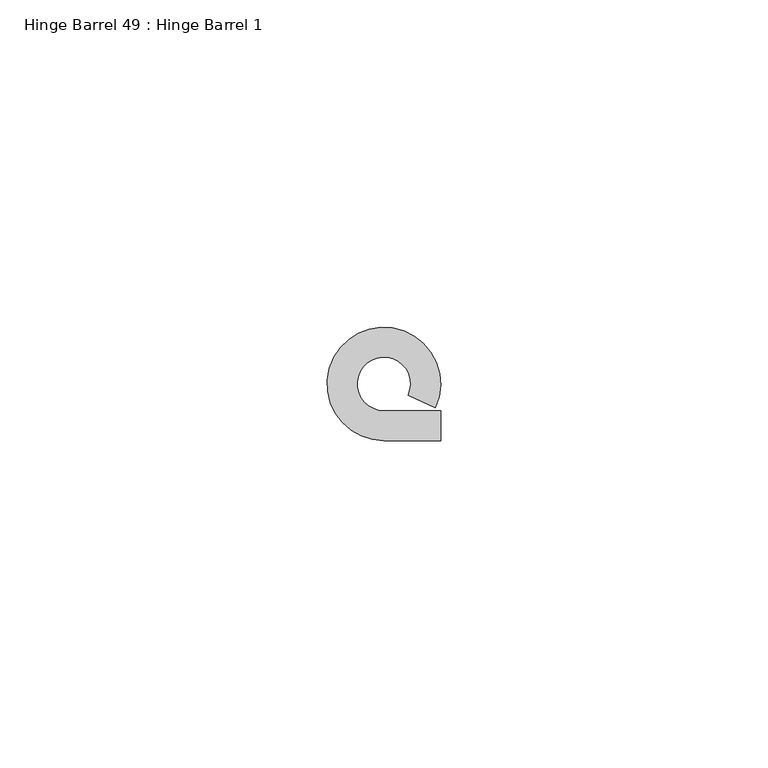
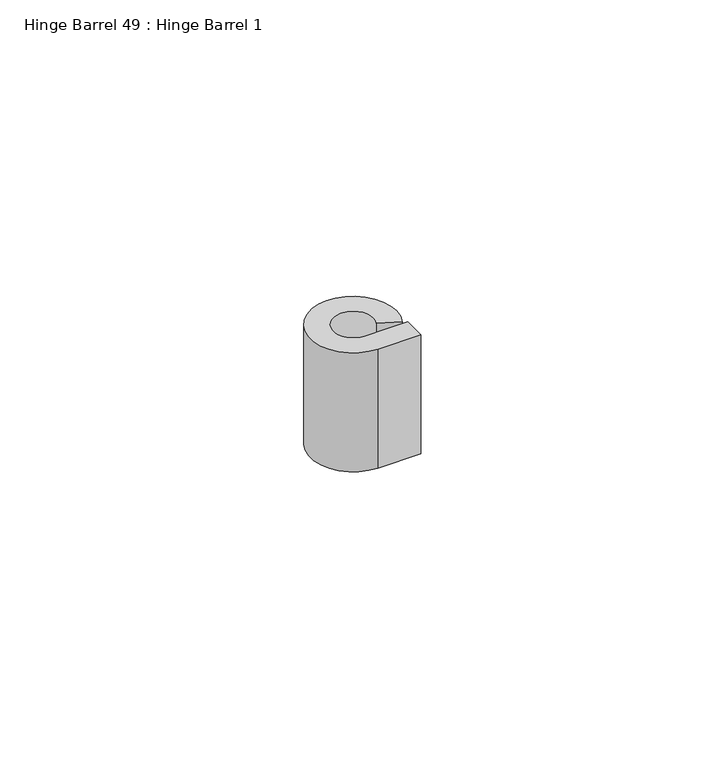
"""IFC4 building model written with IfcOpenShell, lengths in millimetres: proxy geometry, Hinge Barrel 49 : Hinge Barrel 1."""

import ifcopenshell
import ifcopenshell.guid

model = None  # the IFC model being written
_history = None  # IfcOwnerHistory: only IFC2X3 demands one
_inside = {}  # id of a spatial element -> (the spatial element, [elements in it])
_under = {}  # id of a project, library or spatial element -> (it, [spatial elements below it])
_declared = {}  # id of a project -> (the project, [libraries it declares])
_typed = {}  # id of a type object -> (the type object, [elements of that type])
_made_of = {}  # id of a material, layer set ... -> (it, [elements and type objects made of it])


def new_model(schema):
    """Start an empty IFC model of exactly this schema.

    Asked for "IFC4X3", IfcOpenShell would pick the latest addendum, in which some entities
    have other attributes; the version numbers below select the first issue.
    IFC2X3 requires an IfcOwnerHistory on every rooted entity: one is made here for all.
    """
    global model, _history
    if schema == "IFC4X3":
        model = ifcopenshell.file(schema_version=(4, 3, 0, 0))
    else:
        model = ifcopenshell.file(schema=schema)
    _inside.clear()
    _under.clear()
    _declared.clear()
    _typed.clear()
    _made_of.clear()
    _history = None
    if model.schema == "IFC2X3":
        org = make("IfcOrganization", Name="unknown")
        user = make(
            "IfcPersonAndOrganization",
            ThePerson=make("IfcPerson", FamilyName="unknown"),
            TheOrganization=org,
        )
        app = make(
            "IfcApplication",
            ApplicationDeveloper=org,
            Version="unknown",
            ApplicationFullName="unknown",
            ApplicationIdentifier="unknown",
        )
        _history = make(
            "IfcOwnerHistory",
            OwningUser=user,
            OwningApplication=app,
            ChangeAction="ADDED",
            CreationDate=0,
        )
    return model


def make(cls, **values):
    """One entity of the class cls with the attributes given. An attribute that is None is left unset."""
    return model.create_entity(
        cls, **{name: value for name, value in values.items() if value is not None}
    )


def rooted(cls, **values):
    """An entity with a GlobalId (a new one), such as an element, a storey or a relation."""
    return make(cls, GlobalId=ifcopenshell.guid.new(), OwnerHistory=_history, **values)


def si_unit(unit_type, name, prefix=None):
    """IfcSIUnit, for example si_unit("LENGTHUNIT", "METRE", prefix="MILLI")."""
    return make("IfcSIUnit", UnitType=unit_type, Prefix=prefix, Name=name)


def assignment(units):
    """IfcUnitAssignment: the units of a project."""
    return None if units is None else make("IfcUnitAssignment", Units=units)


def point(xyz):
    """IfcCartesianPoint."""
    return None if xyz is None else make("IfcCartesianPoint", Coordinates=xyz)


def direction(xyz):
    """IfcDirection."""
    return None if xyz is None else make("IfcDirection", DirectionRatios=xyz)


def frame(location, z_axis=None, x_axis=None):
    """IfcAxis2Placement3D, a coordinate frame: its origin and axes. An axis left out is left unset."""
    return make(
        "IfcAxis2Placement3D",
        Location=point(location),
        Axis=direction(z_axis),
        RefDirection=direction(x_axis),
    )


def frame_2d(location, x_axis=None):
    """IfcAxis2Placement2D, a coordinate frame in the plane: its origin and x axis."""
    return make(
        "IfcAxis2Placement2D", Location=point(location), RefDirection=direction(x_axis)
    )


def origin():
    """The frame at (0, 0, 0) with its axes left unset."""
    return frame((0.0, 0.0, 0.0))


def place(relative_to, where):
    """IfcLocalPlacement: puts the frame where relative to a parent placement (None: the world)."""
    return make(
        "IfcLocalPlacement", PlacementRelTo=relative_to, RelativePlacement=where
    )


def context(
    kind, dimensions, precision=None, world=None, true_north=None, identifier=None
):
    """IfcGeometricRepresentationContext, for example the 3D "Model" context."""
    return make(
        "IfcGeometricRepresentationContext",
        ContextIdentifier=identifier,
        ContextType=kind,
        CoordinateSpaceDimension=dimensions,
        Precision=precision,
        WorldCoordinateSystem=world,
        TrueNorth=true_north,
    )


def project(units=None, contexts=None):
    """IfcProject with its units and contexts."""
    return rooted(
        "IfcProject",
        Name="project",
        RepresentationContexts=contexts,
        UnitsInContext=assignment(units),
    )


def spatial(cls, under=None, at=None, **own):
    """A site, building, storey or space (cls), placed at a placement, below another one or the project."""
    s = rooted(cls, ObjectPlacement=at, **own)
    if under is not None:
        _under.setdefault(under.id(), (under, []))[1].append(s)
    return s


def polyline(points):
    """IfcPolyline through the points."""
    return make("IfcPolyline", Points=[point(p) for p in points])


def circle_curve(where, radius):
    """IfcCircle in the frame where."""
    return make("IfcCircle", Position=where, Radius=radius)


def trimmed(basis, trim1, trim2, sense, master):
    """IfcTrimmedCurve: the piece of a basis curve between two trims."""
    return make(
        "IfcTrimmedCurve",
        BasisCurve=basis,
        Trim1=trim1,
        Trim2=trim2,
        SenseAgreement=sense,
        MasterRepresentation=master,
    )


def segment(curve, same_sense, transition):
    """IfcCompositeCurveSegment."""
    return make(
        "IfcCompositeCurveSegment",
        Transition=transition,
        SameSense=same_sense,
        ParentCurve=curve,
    )


def composite_curve(segments, self_intersect=None):
    """IfcCompositeCurve: segments joined end to end."""
    return make("IfcCompositeCurve", Segments=segments, SelfIntersect=self_intersect)


def outline(outer, holes=None, kind="AREA"):
    """IfcArbitraryClosedProfileDef: a profile drawn as a closed curve; with holes, ...WithVoids."""
    if holes is None:
        return make("IfcArbitraryClosedProfileDef", ProfileType=kind, OuterCurve=outer)
    return make(
        "IfcArbitraryProfileDefWithVoids",
        ProfileType=kind,
        OuterCurve=outer,
        InnerCurves=holes,
    )


def extrude(swept, where, along, depth):
    """IfcExtrudedAreaSolid: the profile swept, set in the frame where, extruded along a direction by depth."""
    return make(
        "IfcExtrudedAreaSolid",
        SweptArea=swept,
        Position=where,
        ExtrudedDirection=direction(along),
        Depth=depth,
    )


def shape(context_of_items, identifier, shape_type, items):
    """IfcShapeRepresentation: the items that make up one representation, for example the "Body"."""
    return make(
        "IfcShapeRepresentation",
        ContextOfItems=context_of_items,
        RepresentationIdentifier=identifier,
        RepresentationType=shape_type,
        Items=items,
    )


def source(mapping_origin, context_of_items, identifier, shape_type, items):
    """IfcRepresentationMap: a shape defined once, which mapped items show again and again."""
    return make(
        "IfcRepresentationMap",
        MappingOrigin=mapping_origin,
        MappedRepresentation=shape(context_of_items, identifier, shape_type, items),
    )


def transform(
    local_origin,
    x_axis=None,
    y_axis=None,
    z_axis=None,
    scale=None,
    scale2=None,
    scale3=None,
    uniform=True,
):
    """IfcCartesianTransformationOperator3D, or its non-uniform kind. x_axis, y_axis, z_axis: its Axis1, 2, 3."""
    if uniform:
        return make(
            "IfcCartesianTransformationOperator3D",
            Axis1=direction(x_axis),
            Axis2=direction(y_axis),
            LocalOrigin=point(local_origin),
            Scale=scale,
            Axis3=direction(z_axis),
        )
    return make(
        "IfcCartesianTransformationOperator3DnonUniform",
        Axis1=direction(x_axis),
        Axis2=direction(y_axis),
        LocalOrigin=point(local_origin),
        Scale=scale,
        Axis3=direction(z_axis),
        Scale2=scale2,
        Scale3=scale3,
    )


def mapped(mapping_source, mapping_target):
    """IfcMappedItem: shows the shape of a source again, moved by a transform."""
    return make(
        "IfcMappedItem", MappingSource=mapping_source, MappingTarget=mapping_target
    )


def made_of(thing, what):
    """Note that an element or type object is made of a material, layer set ...; save() writes the relation."""
    if what is not None:
        _made_of.setdefault(what.id(), (what, []))[1].append(thing)
    return thing


def element(
    cls,
    number,
    at=None,
    inside=None,
    cuts=None,
    type_object=None,
    material=None,
    context=None,
    identifier="Body",
    shape_type=None,
    held_by="IfcProductDefinitionShape",
    body=None,
    shapes=None,
    **own,
):
    """One element of the class cls, such as IfcWall. Its Tag is "e" and its number.

    at: its placement. inside: the storey or other place that contains it. cuts: it is an
    opening in that element (IfcRelVoidsElement). A single representation is given by context,
    identifier, shape_type and body (its items); several are given by shapes. held_by: the class
    of the entity that holds the representations. save() writes the other relations.
    """
    e = rooted(cls, Tag="e%d" % number, ObjectPlacement=at, **own)
    if body is not None:
        shapes = [shape(context, identifier, shape_type, body)]
    if shapes is not None:
        e.Representation = make(held_by, Representations=shapes)
    if inside is not None:
        _inside.setdefault(inside.id(), (inside, []))[1].append(e)
    if cuts is not None:
        rooted(
            "IfcRelVoidsElement", RelatingBuildingElement=cuts, RelatedOpeningElement=e
        )
    if type_object is not None:
        _typed.setdefault(type_object.id(), (type_object, []))[1].append(e)
    return made_of(e, material)


def aggregate(whole, parts):
    """IfcRelAggregates: a whole, such as a stair, and the parts it consists of."""
    return rooted("IfcRelAggregates", RelatingObject=whole, RelatedObjects=parts)


def save(model, path):
    """Write the relations noted so far, then the file.

    IfcRelAggregates (storeys below a building ...), IfcRelContainedInSpatialStructure (elements
    in a storey), IfcRelDefinesByType, IfcRelAssociatesMaterial and IfcRelDeclares: one each for
    every whole, place, type object, material and project.
    """
    for whole, parts in _under.values():
        aggregate(whole, parts)
    for where, things in _inside.values():
        rooted(
            "IfcRelContainedInSpatialStructure",
            RelatedElements=things,
            RelatingStructure=where,
        )
    for kind, things in _typed.values():
        rooted("IfcRelDefinesByType", RelatedObjects=things, RelatingType=kind)
    for what, things in _made_of.values():
        rooted("IfcRelAssociatesMaterial", RelatedObjects=things, RelatingMaterial=what)
    for by, libraries in _declared.values():
        rooted("IfcRelDeclares", RelatingContext=by, RelatedDefinitions=libraries)
    model.write(path)


def hinge_barrel_49_hinge_barrel_1_b6c159eb(model_context):
    return source(origin(), model_context, "Body", "SweptSolid", [
        extrude(outline(composite_curve([segment(polyline([(587323.2214739, -534104.7943841), (587327.7934739, -534104.7943841), (587327.7934739, -534109.3584466), (587319.1320739, -534109.3584466)]), True, "CONTINUOUS"), segment(trimmed(circle_curve(frame_2d((587319.1320739, -534100.7049841)), 8.6534625), [point((587319.1320739, -534109.3584466))], [point((587326.986084, -534104.3377433))], False, "CARTESIAN"), True, "CONTINUOUS"), segment(polyline([(587326.986084, -534104.3377433), (587322.8436736, -534102.421731)]), True, "CONTINUOUS"), segment(trimmed(circle_curve(frame_2d((587319.1320739, -534100.7049841)), 4.0894), [point((587322.8436736, -534102.421731))], [point((587319.1320739, -534104.7943841))], True, "CARTESIAN"), True, "CONTINUOUS"), segment(polyline([(587319.1320739, -534104.7943841), (587323.2214739, -534104.7943841)]), True, "CONTINUOUS")], self_intersect=False)), frame((0.0, 0.0, 1123.95), z_axis=(0.0, 0.0, 1.0), x_axis=(1.0, 0.0, 0.0)), (0.0, 0.0, 1.0), 25.4),
    ])


if __name__ == "__main__":
    model = new_model("IFC4")
    model_context = context("Model", 3, world=origin())
    ifc_project = project(units=[si_unit("LENGTHUNIT", "METRE", prefix="MILLI")], contexts=[model_context])
    site = spatial("IfcSite", under=ifc_project)
    building = spatial("IfcBuilding", under=site)
    placement = place(None, origin())
    hinge_barrel_49_hinge_barrel_1_shape = hinge_barrel_49_hinge_barrel_1_b6c159eb(model_context)
    element("IfcBuildingElementProxy", 1, Name="Hinge Barrel 49 : Hinge Barrel 1", ObjectType="Hinge Barrel 49 : Hinge Barrel 1", at=placement, inside=building, context=model_context, shape_type="MappedRepresentation", body=[
        mapped(hinge_barrel_49_hinge_barrel_1_shape, transform((0.0, 0.0, 0.0), x_axis=(1.0, 0.0, 0.0), y_axis=(0.0, 1.0, 0.0), z_axis=(0.0, 0.0, 1.0))),
    ])
    save(model, "model.ifc")

# Revit data of these elements
# Element 1 (IfcBuildingElementProxy, "Hinge Barrel 49 : Hinge Barrel 1")
#   Materials on its faces: "6\"X6\" WELD-ON STL BUTT HINGE"
# Materials
#   "6\"X6\" WELD-ON STL BUTT HINGE": class "Metal", colour RGB 189 187 185, transparency 0, Description = "Carbon steel", Cost = 0
